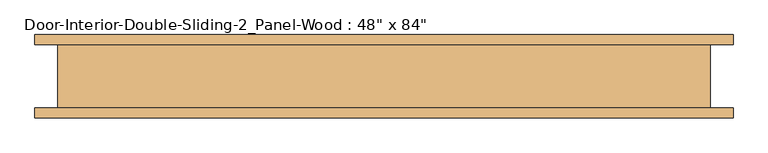
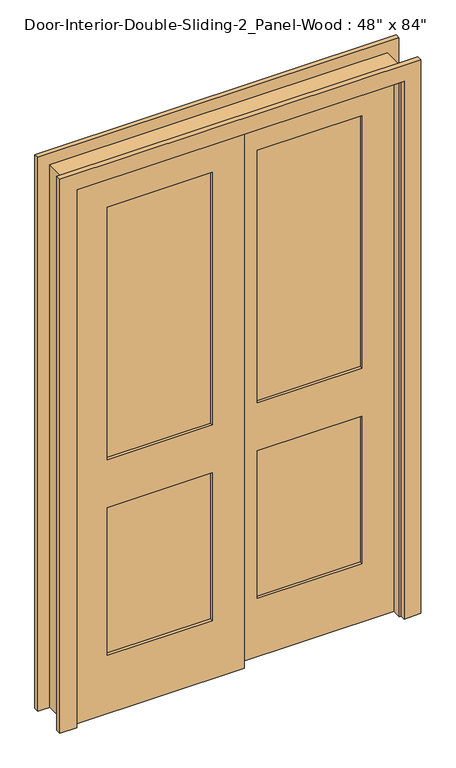
"""IFC4 building model written with IfcOpenShell, lengths in millimetres: door geometry."""

from ifc_helpers import new_model, si_unit, frame, origin, place, context, project, spatial, polyline, outline, extrude, source, transform, mapped, element, save


def door_b8c0c601(model_context):
    return source(origin(), model_context, "Body", "SweptSolid", [
        extrude(outline(polyline([(488.95, -0.5291667), (488.95, -12.1708333), (95.25, -12.1708333), (95.25, -0.5291667), (488.95, -0.5291667)])), frame((0.0, 0.0, 1009.65), z_axis=(0.0, 0.0, 1.0), x_axis=(1.0, 0.0, 0.0)), (0.0, 0.0, 1.0), 1004.8875),
        extrude(outline(polyline([(488.95, -0.5291667), (488.95, -12.1708333), (95.25, -12.1708333), (95.25, -0.5291667), (488.95, -0.5291667)])), frame((0.0, 0.0, 231.775), z_axis=(0.0, 0.0, 1.0), x_axis=(1.0, 0.0, 0.0)), (0.0, 0.0, 1.0), 587.375),
        extrude(outline(polyline([(2133.6, -25.4), (0.0, -25.4), (0.0, 609.6), (2133.6, 609.6), (2133.6, -25.4)]), holes=[polyline([(2014.5375, 95.25), (2014.5375, 488.95), (1009.65, 488.95), (1009.65, 95.25), (2014.5375, 95.25)]), polyline([(819.15, 95.25), (819.15, 488.95), (231.775, 488.95), (231.775, 95.25), (819.15, 95.25)])]), frame((0.0, -23.8125, 0.0), z_axis=(0.0, 1.0, 0.0), x_axis=(0.0, 0.0, 1.0)), (0.0, 0.0, 1.0), 34.925),
        extrude(outline(polyline([(-95.25, -35.4541667), (-95.25, -47.0958333), (-488.95, -47.0958333), (-488.95, -35.4541667), (-95.25, -35.4541667)])), frame((0.0, 0.0, 1009.65), z_axis=(0.0, 0.0, 1.0), x_axis=(1.0, 0.0, 0.0)), (0.0, 0.0, 1.0), 1004.8875),
        extrude(outline(polyline([(-95.25, -35.4541667), (-95.25, -47.0958333), (-488.95, -47.0958333), (-488.95, -35.4541667), (-95.25, -35.4541667)])), frame((0.0, 0.0, 231.775), z_axis=(0.0, 0.0, 1.0), x_axis=(1.0, 0.0, 0.0)), (0.0, 0.0, 1.0), 587.375),
        extrude(outline(polyline([(2133.6, -609.6), (0.0, -609.6), (0.0, 25.4), (2133.6, 25.4), (2133.6, -609.6)]), holes=[polyline([(2014.5375, -488.95), (2014.5375, -95.25), (1009.65, -95.25), (1009.65, -488.95), (2014.5375, -488.95)]), polyline([(819.15, -488.95), (819.15, -95.25), (231.775, -95.25), (231.775, -488.95), (819.15, -488.95)])]), frame((0.0, -58.7375, 0.0), z_axis=(0.0, 1.0, 0.0), x_axis=(0.0, 0.0, 1.0)), (0.0, 0.0, 1.0), 34.925),
        extrude(outline(polyline([(0.0, 635.0), (2159.0, 635.0), (2159.0, -635.0), (0.0, -635.0), (0.0, -609.6), (2133.6, -609.6), (2133.6, 609.6), (0.0, 609.6), (0.0, 635.0)])), frame((0.0, -58.7375, 0.0), z_axis=(0.0, 1.0, 0.0), x_axis=(0.0, 0.0, 1.0)), (0.0, 0.0, 1.0), 123.825),
        extrude(outline(polyline([(0.0, 679.45), (2203.45, 679.45), (2203.45, -679.45), (0.0, -679.45), (0.0, -615.95), (2139.95, -615.95), (2139.95, 615.95), (0.0, 615.95), (0.0, 679.45)])), frame((0.0, 65.0875, 0.0), z_axis=(0.0, 1.0, 0.0), x_axis=(0.0, 0.0, 1.0)), (0.0, 0.0, 1.0), 19.05),
        extrude(outline(polyline([(0.0, 679.45), (2203.45, 679.45), (2203.45, -679.45), (0.0, -679.45), (0.0, -615.95), (2139.95, -615.95), (2139.95, 615.95), (0.0, 615.95), (0.0, 679.45)])), frame((0.0, -77.7875, 0.0), z_axis=(0.0, 1.0, 0.0), x_axis=(0.0, 0.0, 1.0)), (0.0, 0.0, 1.0), 19.05),
    ])


if __name__ == "__main__":
    model = new_model("IFC4")
    model_context = context("Model", 3, world=origin())
    ifc_project = project(units=[si_unit("LENGTHUNIT", "METRE", prefix="MILLI")], contexts=[model_context])
    site = spatial("IfcSite", under=ifc_project)
    building = spatial("IfcBuilding", under=site)
    placement = place(None, origin())
    door_shape = door_b8c0c601(model_context)
    element("IfcDoor", 1, ObjectType="Door-Interior-Double-Sliding-2_Panel-Wood : 48\" x 84\"", at=placement, inside=building, context=model_context, shape_type="MappedRepresentation", body=[
        mapped(door_shape, transform((0.0, 0.0, 0.0), x_axis=(1.0, 0.0, 0.0), y_axis=(0.0, 1.0, 0.0), z_axis=(0.0, 0.0, 1.0))),
    ])
    save(model, "model.ifc")

# Revit data of these elements
# Type "Door-Interior-Double-Sliding-2_Panel-Wood : 48\" x 84\""
#   Type Mark = "21"
#   Assembly Code = "C1020300"
#   Analytic Construction = "Wooden"
#   Top Rail = 0' - 4 11/16"
#   Thickness = 0' - 1 3/8"
#   Thermal Resistance (R) = 2.5876 (h·ft²·°F)/BTU
#   Stiles = 0' - 4 3/4"
#   Rough Width = 4' - 2"
#   Rough Height = 7' - 1"
#   Lock Rail = 0' - 7 1/2"
#   Height = 7' - 0"
#   Width = 4' - 0"
#   Heat Transfer Coefficient (U) = 0.3865 BTU/(h·ft²·°F)
#   Bottom Rail = 0' - 9 1/8"
#   Trim Material = Cherry
#   Panel Material = Cherry
#   Frame Material = Cherry
#   Visual Light Transmittance = 0
#   Solar Heat Gain Coefficient = 0
#   Wall Closure = (empty or 0)
#   Function = (empty or 0)
# Element 1 (IfcDoor, "Door-Interior-Double-Sliding-2_Panel-Wood : 48\" x 84\"")
#   Materials on its faces: "Cherry"
# Materials
#   "Cherry": class "Wood", colour RGB 226 177 128, transparency 0, Description = "Prunus Serotina", Cost = 0
